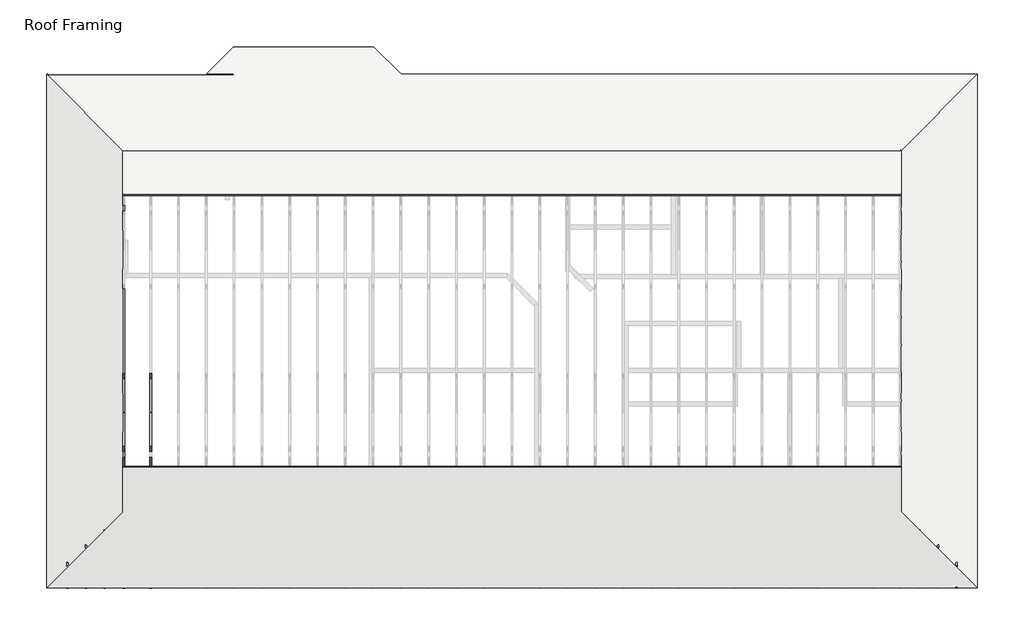
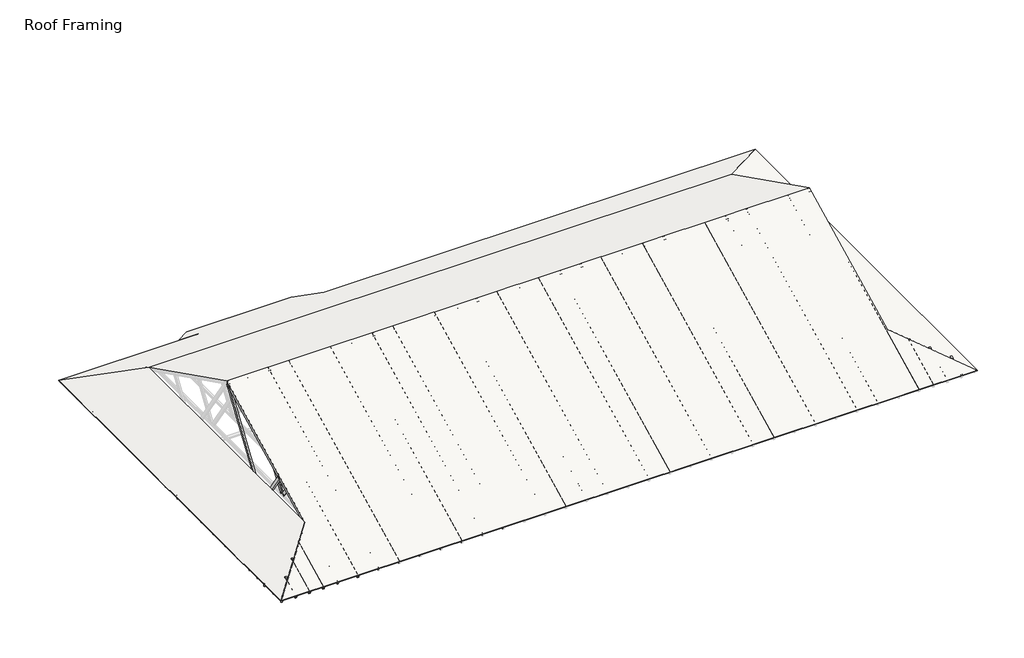
# One storey, part 1 of 7: 42 beams, 4 members, 4 roofs.
"""IFC4 building model written with IfcOpenShell, lengths in millimetres."""

import ifcopenshell
import ifcopenshell.guid

model = None  # the IFC model being written
_history = None  # IfcOwnerHistory: only IFC2X3 demands one
_inside = {}  # id of a spatial element -> (the spatial element, [elements in it])
_under = {}  # id of a project, library or spatial element -> (it, [spatial elements below it])
_declared = {}  # id of a project -> (the project, [libraries it declares])
_typed = {}  # id of a type object -> (the type object, [elements of that type])
_made_of = {}  # id of a material, layer set ... -> (it, [elements and type objects made of it])


def new_model(schema):
    """Start an empty IFC model of exactly this schema.

    Asked for "IFC4X3", IfcOpenShell would pick the latest addendum, in which some entities
    have other attributes; the version numbers below select the first issue.
    IFC2X3 requires an IfcOwnerHistory on every rooted entity: one is made here for all.
    """
    global model, _history
    if schema == "IFC4X3":
        model = ifcopenshell.file(schema_version=(4, 3, 0, 0))
    else:
        model = ifcopenshell.file(schema=schema)
    _inside.clear()
    _under.clear()
    _declared.clear()
    _typed.clear()
    _made_of.clear()
    _history = None
    if model.schema == "IFC2X3":
        org = make("IfcOrganization", Name="unknown")
        user = make(
            "IfcPersonAndOrganization",
            ThePerson=make("IfcPerson", FamilyName="unknown"),
            TheOrganization=org,
        )
        app = make(
            "IfcApplication",
            ApplicationDeveloper=org,
            Version="unknown",
            ApplicationFullName="unknown",
            ApplicationIdentifier="unknown",
        )
        _history = make(
            "IfcOwnerHistory",
            OwningUser=user,
            OwningApplication=app,
            ChangeAction="ADDED",
            CreationDate=0,
        )
    return model


def make(cls, **values):
    """One entity of the class cls with the attributes given. An attribute that is None is left unset."""
    return model.create_entity(
        cls, **{name: value for name, value in values.items() if value is not None}
    )


def rooted(cls, **values):
    """An entity with a GlobalId (a new one), such as an element, a storey or a relation."""
    return make(cls, GlobalId=ifcopenshell.guid.new(), OwnerHistory=_history, **values)


def si_unit(unit_type, name, prefix=None):
    """IfcSIUnit, for example si_unit("LENGTHUNIT", "METRE", prefix="MILLI")."""
    return make("IfcSIUnit", UnitType=unit_type, Prefix=prefix, Name=name)


def assignment(units):
    """IfcUnitAssignment: the units of a project."""
    return None if units is None else make("IfcUnitAssignment", Units=units)


def point(xyz):
    """IfcCartesianPoint."""
    return None if xyz is None else make("IfcCartesianPoint", Coordinates=xyz)


def direction(xyz):
    """IfcDirection."""
    return None if xyz is None else make("IfcDirection", DirectionRatios=xyz)


def frame(location, z_axis=None, x_axis=None):
    """IfcAxis2Placement3D, a coordinate frame: its origin and axes. An axis left out is left unset."""
    return make(
        "IfcAxis2Placement3D",
        Location=point(location),
        Axis=direction(z_axis),
        RefDirection=direction(x_axis),
    )


def origin():
    """The frame at (0, 0, 0) with its axes left unset."""
    return frame((0.0, 0.0, 0.0))


def place(relative_to, where):
    """IfcLocalPlacement: puts the frame where relative to a parent placement (None: the world)."""
    return make(
        "IfcLocalPlacement", PlacementRelTo=relative_to, RelativePlacement=where
    )


def context(
    kind, dimensions, precision=None, world=None, true_north=None, identifier=None
):
    """IfcGeometricRepresentationContext, for example the 3D "Model" context."""
    return make(
        "IfcGeometricRepresentationContext",
        ContextIdentifier=identifier,
        ContextType=kind,
        CoordinateSpaceDimension=dimensions,
        Precision=precision,
        WorldCoordinateSystem=world,
        TrueNorth=true_north,
    )


def project(units=None, contexts=None):
    """IfcProject with its units and contexts."""
    return rooted(
        "IfcProject",
        Name="project",
        RepresentationContexts=contexts,
        UnitsInContext=assignment(units),
    )


def spatial(cls, under=None, at=None, **own):
    """A site, building, storey or space (cls), placed at a placement, below another one or the project."""
    s = rooted(cls, ObjectPlacement=at, **own)
    if under is not None:
        _under.setdefault(under.id(), (under, []))[1].append(s)
    return s


def polyline(points):
    """IfcPolyline through the points."""
    return make("IfcPolyline", Points=[point(p) for p in points])


def outline(outer, holes=None, kind="AREA"):
    """IfcArbitraryClosedProfileDef: a profile drawn as a closed curve; with holes, ...WithVoids."""
    if holes is None:
        return make("IfcArbitraryClosedProfileDef", ProfileType=kind, OuterCurve=outer)
    return make(
        "IfcArbitraryProfileDefWithVoids",
        ProfileType=kind,
        OuterCurve=outer,
        InnerCurves=holes,
    )


def extrude(swept, where, along, depth):
    """IfcExtrudedAreaSolid: the profile swept, set in the frame where, extruded along a direction by depth."""
    return make(
        "IfcExtrudedAreaSolid",
        SweptArea=swept,
        Position=where,
        ExtrudedDirection=direction(along),
        Depth=depth,
    )


def faces_of(points, faces, orient=None, outer=None):
    """IfcFace entities. A face is a list of loops; a loop is a list of indices into points, from 0.

    orient and outer hold one flag for each loop. By default every Orientation is true, the
    first loop of a face is its IfcFaceOuterBound and the others are IfcFaceBound.
    """
    made = []
    for i, loops in enumerate(faces):
        bounds = []
        for j, loop in enumerate(loops):
            is_outer = j == 0 if outer is None else outer[i][j]
            bounds.append(
                make(
                    "IfcFaceOuterBound" if is_outer else "IfcFaceBound",
                    Bound=make("IfcPolyLoop", Polygon=[points[k] for k in loop]),
                    Orientation=True if orient is None else orient[i][j],
                )
            )
        made.append(make("IfcFace", Bounds=bounds))
    return made


def faceted_brep(points, faces, orient=None, outer=None, voids=None):
    """IfcFacetedBrep: a solid bounded by flat faces; with voids (closed shells), ...WithVoids."""
    shared = [point(p) for p in points]
    hull = make("IfcClosedShell", CfsFaces=faces_of(shared, faces, orient, outer))
    if voids is None:
        return make("IfcFacetedBrep", Outer=hull)
    return make(
        "IfcFacetedBrepWithVoids",
        Outer=hull,
        Voids=[
            make(cls, CfsFaces=faces_of(shared, fs, o, b)) for cls, fs, o, b in voids
        ],
    )


def shape(context_of_items, identifier, shape_type, items):
    """IfcShapeRepresentation: the items that make up one representation, for example the "Body"."""
    return make(
        "IfcShapeRepresentation",
        ContextOfItems=context_of_items,
        RepresentationIdentifier=identifier,
        RepresentationType=shape_type,
        Items=items,
    )


def source(mapping_origin, context_of_items, identifier, shape_type, items):
    """IfcRepresentationMap: a shape defined once, which mapped items show again and again."""
    return make(
        "IfcRepresentationMap",
        MappingOrigin=mapping_origin,
        MappedRepresentation=shape(context_of_items, identifier, shape_type, items),
    )


def transform(
    local_origin,
    x_axis=None,
    y_axis=None,
    z_axis=None,
    scale=None,
    scale2=None,
    scale3=None,
    uniform=True,
):
    """IfcCartesianTransformationOperator3D, or its non-uniform kind. x_axis, y_axis, z_axis: its Axis1, 2, 3."""
    if uniform:
        return make(
            "IfcCartesianTransformationOperator3D",
            Axis1=direction(x_axis),
            Axis2=direction(y_axis),
            LocalOrigin=point(local_origin),
            Scale=scale,
            Axis3=direction(z_axis),
        )
    return make(
        "IfcCartesianTransformationOperator3DnonUniform",
        Axis1=direction(x_axis),
        Axis2=direction(y_axis),
        LocalOrigin=point(local_origin),
        Scale=scale,
        Axis3=direction(z_axis),
        Scale2=scale2,
        Scale3=scale3,
    )


def mapped(mapping_source, mapping_target):
    """IfcMappedItem: shows the shape of a source again, moved by a transform."""
    return make(
        "IfcMappedItem", MappingSource=mapping_source, MappingTarget=mapping_target
    )


def made_of(thing, what):
    """Note that an element or type object is made of a material, layer set ...; save() writes the relation."""
    if what is not None:
        _made_of.setdefault(what.id(), (what, []))[1].append(thing)
    return thing


def element(
    cls,
    number,
    at=None,
    inside=None,
    cuts=None,
    type_object=None,
    material=None,
    context=None,
    identifier="Body",
    shape_type=None,
    held_by="IfcProductDefinitionShape",
    body=None,
    shapes=None,
    **own,
):
    """One element of the class cls, such as IfcWall. Its Tag is "e" and its number.

    at: its placement. inside: the storey or other place that contains it. cuts: it is an
    opening in that element (IfcRelVoidsElement). A single representation is given by context,
    identifier, shape_type and body (its items); several are given by shapes. held_by: the class
    of the entity that holds the representations. save() writes the other relations.
    """
    e = rooted(cls, Tag="e%d" % number, ObjectPlacement=at, **own)
    if body is not None:
        shapes = [shape(context, identifier, shape_type, body)]
    if shapes is not None:
        e.Representation = make(held_by, Representations=shapes)
    if inside is not None:
        _inside.setdefault(inside.id(), (inside, []))[1].append(e)
    if cuts is not None:
        rooted(
            "IfcRelVoidsElement", RelatingBuildingElement=cuts, RelatedOpeningElement=e
        )
    if type_object is not None:
        _typed.setdefault(type_object.id(), (type_object, []))[1].append(e)
    return made_of(e, material)


def aggregate(whole, parts):
    """IfcRelAggregates: a whole, such as a stair, and the parts it consists of."""
    return rooted("IfcRelAggregates", RelatingObject=whole, RelatedObjects=parts)


def save(model, path):
    """Write the relations noted so far, then the file.

    IfcRelAggregates (storeys below a building ...), IfcRelContainedInSpatialStructure (elements
    in a storey), IfcRelDefinesByType, IfcRelAssociatesMaterial and IfcRelDeclares: one each for
    every whole, place, type object, material and project.
    """
    for whole, parts in _under.values():
        aggregate(whole, parts)
    for where, things in _inside.values():
        rooted(
            "IfcRelContainedInSpatialStructure",
            RelatedElements=things,
            RelatingStructure=where,
        )
    for kind, things in _typed.values():
        rooted("IfcRelDefinesByType", RelatedObjects=things, RelatingType=kind)
    for what, things in _made_of.values():
        rooted("IfcRelAssociatesMaterial", RelatedObjects=things, RelatingMaterial=what)
    for by, libraries in _declared.values():
        rooted("IfcRelDeclares", RelatingContext=by, RelatedDefinitions=libraries)
    model.write(path)


def dimension_lumber_3c164bda(model_context):
    return source(origin(), model_context, "Body", "SweptSolid", [
        extrude(outline(polyline([(4638.675, -19.05), (-5762.625, -19.05), (-5762.625, 19.05), (4638.675, 19.05), (4638.675, -19.05)])), frame((0.0, 0.0, -44.45), z_axis=(0.0, 0.0, 1.0), x_axis=(1.0, 0.0, 0.0)), (0.0, 0.0, 1.0), 88.9),
    ])


def dimension_lumber_70fa0837(model_context):
    return source(origin(), model_context, "Body", "SweptSolid", [
        extrude(outline(polyline([(1250.4988621, 19.05), (1250.4988621, -19.05), (-1214.6940206, -19.05), (-1214.6940206, 19.05), (1250.4988621, 19.05)])), frame((0.0, 0.0, -44.45), z_axis=(0.0, 0.0, 1.0), x_axis=(1.0, 0.0, 0.0)), (0.0, 0.0, 1.0), 88.9),
    ])


def dimension_lumber_c8f8d63a(model_context):
    return source(origin(), model_context, "Body", "SweptSolid", [
        extrude(outline(polyline([(5118.89375, 44.45), (5118.89375, -44.45), (-5118.89375, -44.45), (-5118.89375, 44.45), (5118.89375, 44.45)])), frame((0.0, 0.0, -19.05), z_axis=(0.0, 0.0, 1.0), x_axis=(1.0, 0.0, 0.0)), (0.0, 0.0, 1.0), 38.1),
    ])


def dimension_lumber_4f6bd669(model_context):
    return source(origin(), model_context, "Body", "SweptSolid", [
        extrude(outline(polyline([(5017.29375, 44.45), (5017.29375, -44.45), (-5144.29375, -44.45), (-5144.29375, 44.45), (5017.29375, 44.45)])), frame((0.0, 0.0, -19.05), z_axis=(0.0, 0.0, 1.0), x_axis=(1.0, 0.0, 0.0)), (0.0, 0.0, 1.0), 38.1),
    ])


model = new_model("IFC4")

# Units and contexts
model_context = context("Model", 3, world=origin())
ifc_project = project(units=[si_unit("LENGTHUNIT", "METRE", prefix="MILLI")], contexts=[model_context])

# Site, building, storey
site = spatial("IfcSite", under=ifc_project)
building = spatial("IfcBuilding", under=site)
storey = spatial("IfcBuildingStorey", under=building, Name="Roof Framing", Elevation=2768.6)

# Beams
placement = place(None, origin())
element("IfcBeam", 1, ObjectType="Dimension Lumber : Roof Lumbers", at=placement, inside=storey, context=model_context, shape_type="SweptSolid", body=[
    extrude(outline(polyline([(-5032.8152251, -4625.6040947), (-5032.8152251, -4663.7040947), (-6240.9027251, -4663.7040947), (-6240.9027251, -4625.6040947), (-5032.8152251, -4625.6040947)])), frame((0.0, 0.0, 2768.6), z_axis=(0.0, 0.0, 1.0), x_axis=(1.0, 0.0, 0.0)), (0.0, 0.0, 1.0), 88.9),
    extrude(outline(polyline([(2768.6, -5032.8152251), (2857.5, -5032.8152251), (2857.5, -6064.1385305), (2769.1179027, -6240.9027251), (2768.6, -6240.9027251), (2768.6, -5032.8152251)])), frame((0.0, -4663.7040947, 0.0), z_axis=(0.0, 1.0, 0.0), x_axis=(0.0, 0.0, 1.0)), (0.0, 0.0, 1.0), 38.1),
])
element("IfcBeam", 2, ObjectType="Dimension Lumber : Roof Lumbers", at=placement, inside=storey, context=model_context, shape_type="SweptSolid", body=[
    extrude(outline(polyline([(-5032.8152251, -4016.0040947), (-5032.8152251, -4054.1040947), (-6240.9027251, -4054.1040947), (-6240.9027251, -4016.0040947), (-5032.8152251, -4016.0040947)])), frame((0.0, 0.0, 2768.6), z_axis=(0.0, 0.0, 1.0), x_axis=(1.0, 0.0, 0.0)), (0.0, 0.0, 1.0), 88.9),
    extrude(outline(polyline([(2768.6, -5032.8152251), (2857.5, -5032.8152251), (2857.5, -6064.1385305), (2769.1179027, -6240.9027251), (2768.6, -6240.9027251), (2768.6, -5032.8152251)])), frame((0.0, -4054.1040947, 0.0), z_axis=(0.0, 1.0, 0.0), x_axis=(0.0, 0.0, 1.0)), (0.0, 0.0, 1.0), 38.1),
])
element("IfcBeam", 3, ObjectType="Dimension Lumber : Roof Lumbers", at=placement, inside=storey, context=model_context, shape_type="SweptSolid", body=[
    extrude(outline(polyline([(-5032.8152251, -3406.4040947), (-5032.8152251, -3444.5040947), (-6240.9027251, -3444.5040947), (-6240.9027251, -3406.4040947), (-5032.8152251, -3406.4040947)])), frame((0.0, 0.0, 2768.6), z_axis=(0.0, 0.0, 1.0), x_axis=(1.0, 0.0, 0.0)), (0.0, 0.0, 1.0), 88.9),
    extrude(outline(polyline([(2768.6, -5032.8152251), (2857.5, -5032.8152251), (2857.5, -6064.1385305), (2769.1179027, -6240.9027251), (2768.6, -6240.9027251), (2768.6, -5032.8152251)])), frame((0.0, -3444.5040947, 0.0), z_axis=(0.0, 1.0, 0.0), x_axis=(0.0, 0.0, 1.0)), (0.0, 0.0, 1.0), 38.1),
])
element("IfcBeam", 4, ObjectType="Dimension Lumber : Roof Lumbers", at=placement, inside=storey, context=model_context, shape_type="SweptSolid", body=[
    extrude(outline(polyline([(-5032.8152251, -2796.8040947), (-5032.8152251, -2834.9040947), (-6240.9027251, -2834.9040947), (-6240.9027251, -2796.8040947), (-5032.8152251, -2796.8040947)])), frame((0.0, 0.0, 2768.6), z_axis=(0.0, 0.0, 1.0), x_axis=(1.0, 0.0, 0.0)), (0.0, 0.0, 1.0), 88.9),
    extrude(outline(polyline([(2768.6, -5032.8152251), (2857.5, -5032.8152251), (2857.5, -6064.1385305), (2769.1179027, -6240.9027251), (2768.6, -6240.9027251), (2768.6, -5032.8152251)])), frame((0.0, -2834.9040947, 0.0), z_axis=(0.0, 1.0, 0.0), x_axis=(0.0, 0.0, 1.0)), (0.0, 0.0, 1.0), 38.1),
])
element("IfcBeam", 5, ObjectType="Dimension Lumber : Roof Lumbers", at=placement, inside=storey, context=model_context, shape_type="SweptSolid", body=[
    extrude(outline(polyline([(-5032.8152251, -2187.2040947), (-5032.8152251, -2225.3040947), (-6240.9027251, -2225.3040947), (-6240.9027251, -2187.2040947), (-5032.8152251, -2187.2040947)])), frame((0.0, 0.0, 2768.6), z_axis=(0.0, 0.0, 1.0), x_axis=(1.0, 0.0, 0.0)), (0.0, 0.0, 1.0), 88.9),
    extrude(outline(polyline([(2768.6, -5032.8152251), (2857.5, -5032.8152251), (2857.5, -6064.1385305), (2769.1179027, -6240.9027251), (2768.6, -6240.9027251), (2768.6, -5032.8152251)])), frame((0.0, -2225.3040947, 0.0), z_axis=(0.0, 1.0, 0.0), x_axis=(0.0, 0.0, 1.0)), (0.0, 0.0, 1.0), 38.1),
])
element("IfcBeam", 6, ObjectType="Dimension Lumber : Roof Lumbers", at=placement, inside=storey, context=model_context, shape_type="SweptSolid", body=[
    extrude(outline(polyline([(-5032.8152251, -1577.6040947), (-5032.8152251, -1615.7040947), (-6240.9027251, -1615.7040947), (-6240.9027251, -1577.6040947), (-5032.8152251, -1577.6040947)])), frame((0.0, 0.0, 2768.6), z_axis=(0.0, 0.0, 1.0), x_axis=(1.0, 0.0, 0.0)), (0.0, 0.0, 1.0), 88.9),
    extrude(outline(polyline([(2768.6, -5032.8152251), (2857.5, -5032.8152251), (2857.5, -6064.1385305), (2769.1179027, -6240.9027251), (2768.6, -6240.9027251), (2768.6, -5032.8152251)])), frame((0.0, -1615.7040947, 0.0), z_axis=(0.0, 1.0, 0.0), x_axis=(0.0, 0.0, 1.0)), (0.0, 0.0, 1.0), 38.1),
])
element("IfcBeam", 7, ObjectType="Dimension Lumber : Roof Lumbers", at=placement, inside=storey, context=model_context, shape_type="SweptSolid", body=[
    extrude(outline(polyline([(-5032.8152251, -968.0040947), (-5032.8152251, -1006.1040947), (-6240.9027251, -1006.1040947), (-6240.9027251, -968.0040947), (-5032.8152251, -968.0040947)])), frame((0.0, 0.0, 2768.6), z_axis=(0.0, 0.0, 1.0), x_axis=(1.0, 0.0, 0.0)), (0.0, 0.0, 1.0), 88.9),
    extrude(outline(polyline([(2768.6, -5032.8152251), (2857.5, -5032.8152251), (2857.5, -6064.1385305), (2769.1179027, -6240.9027251), (2768.6, -6240.9027251), (2768.6, -5032.8152251)])), frame((0.0, -1006.1040947, 0.0), z_axis=(0.0, 1.0, 0.0), x_axis=(0.0, 0.0, 1.0)), (0.0, 0.0, 1.0), 38.1),
])
element("IfcBeam", 8, ObjectType="Dimension Lumber : Roof Lumbers", at=placement, inside=storey, context=model_context, shape_type="SweptSolid", body=[
    extrude(outline(polyline([(-5032.8152251, -358.4040947), (-5032.8152251, -396.5040947), (-6240.9027251, -396.5040947), (-6240.9027251, -358.4040947), (-5032.8152251, -358.4040947)])), frame((0.0, 0.0, 2768.6), z_axis=(0.0, 0.0, 1.0), x_axis=(1.0, 0.0, 0.0)), (0.0, 0.0, 1.0), 88.9),
    extrude(outline(polyline([(2768.6, -5032.8152251), (2857.5, -5032.8152251), (2857.5, -6064.1385305), (2769.1179027, -6240.9027251), (2768.6, -6240.9027251), (2768.6, -5032.8152251)])), frame((0.0, -396.5040947, 0.0), z_axis=(0.0, 1.0, 0.0), x_axis=(0.0, 0.0, 1.0)), (0.0, 0.0, 1.0), 38.1),
])
element("IfcBeam", 9, ObjectType="Dimension Lumber : Roof Lumbers", at=placement, inside=storey, context=model_context, shape_type="Brep", body=[
    faceted_brep([(-5458.2652251, -5041.9472419, 3273.9083007), (-5420.1652251, -5041.9472419, 3273.9083007), (-5420.1652251, -5002.1899532, 3194.3937234), (-5458.2652251, -5002.1899532, 3194.3937234), (-5458.2652251, -6329.0380921, 2630.3628756), (-5458.2652251, -6289.2808035, 2550.8482983), (-5420.1652251, -6289.2808035, 2550.8482983), (-5420.1652251, -6329.0380921, 2630.3628756)], [[[0, 1, 2, 3]], [[4, 5, 6, 7]], [[1, 0, 4, 7]], [[2, 1, 7, 6]], [[3, 2, 6, 5]], [[0, 3, 5, 4]]]),
    faceted_brep([(-5458.2652251, -6329.0380921, 2630.3628756), (-5458.2652251, -6289.2808035, 2550.8482983), (-5420.1652251, -6289.2808035, 2550.8482983), (-5420.1652251, -6329.0380921, 2630.3628756), (-5458.2652251, -5097.0448631, 3146.9662685), (-5458.2652251, -5097.0448631, 3246.3594901), (-5420.1652251, -5058.9448631, 3166.0162685), (-5420.1652251, -5058.9448631, 3265.4094901)], [[[0, 1, 2, 3]], [[4, 1, 0, 5]], [[6, 2, 1, 4]], [[7, 3, 2, 6]], [[5, 0, 3, 7]], [[5, 7, 6, 4]]]),
    faceted_brep([(-5458.2652251, -6329.0380921, 2630.3628756), (-5458.2652251, -6296.1597793, 2564.60625), (-5420.1652251, -6296.1597793, 2564.60625), (-5420.1652251, -6329.0380921, 2630.3628756), (-5458.2652251, -5097.0448631, 3146.9662685), (-5458.2652251, -6261.7649001, 2564.60625), (-5458.2652251, -5097.0448631, 3246.3594901), (-5420.1652251, -5058.9448631, 3265.4094901), (-5420.1652251, -6261.7649001, 2564.60625), (-5420.1652251, -5058.9448631, 3166.0162685)], [[[0, 1, 2, 3]], [[4, 5, 1, 0, 6]], [[7, 3, 2, 8, 9]], [[6, 0, 3, 7]], [[9, 8, 5, 4]], [[6, 7, 9, 4]], [[2, 1, 5, 8]]]),
    faceted_brep([(-5458.2652251, -5097.0448631, 3146.9662685), (-5458.2652251, -6261.7649001, 2564.60625), (-5458.2652251, -6282.9540947, 2564.60625), (-5458.2652251, -6282.9540947, 2653.4048743), (-5458.2652251, -5097.0448631, 3246.3594901), (-5420.1652251, -5058.9448631, 3166.0162685), (-5420.1652251, -6261.7649001, 2564.60625), (-5420.1652251, -6282.9540947, 2564.60625), (-5420.1652251, -6282.9540947, 2653.4048743), (-5420.1652251, -5058.9448631, 3265.4094901)], [[[0, 1, 2, 3, 4]], [[5, 6, 1, 0]], [[2, 1, 6, 7]], [[4, 3, 8, 9]], [[4, 9, 5, 0]], [[9, 8, 7, 6, 5]], [[3, 2, 7, 8]]]),
])
element("IfcBeam", 10, ObjectType="Dimension Lumber : Roof Lumbers", at=placement, inside=storey, context=model_context, shape_type="Brep", body=[
    faceted_brep([(-5864.6652251, -5385.152618, 3102.3056127), (-5826.5652251, -5385.152618, 3102.3056127), (-5826.5652251, -5345.3953294, 3022.7910354), (-5864.6652251, -5345.3953294, 3022.7910354), (-5864.6652251, -6329.0380921, 2630.3628756), (-5864.6652251, -6289.2808035, 2550.8482983), (-5826.5652251, -6289.2808035, 2550.8482983), (-5826.5652251, -6329.0380921, 2630.3628756)], [[[0, 1, 2, 3]], [[4, 5, 6, 7]], [[1, 0, 4, 7]], [[2, 1, 7, 6]], [[3, 2, 6, 5]], [[0, 3, 5, 4]]]),
    faceted_brep([(-5864.6652251, -6329.0380921, 2630.3628756), (-5864.6652251, -6289.2808035, 2550.8482983), (-5826.5652251, -6289.2808035, 2550.8482983), (-5826.5652251, -6329.0380921, 2630.3628756), (-5864.6652251, -5503.4448631, 2943.7662685), (-5864.6652251, -5503.4448631, 3043.1594901), (-5826.5652251, -5465.3448631, 2962.8162685), (-5826.5652251, -5465.3448631, 3062.2094901)], [[[0, 1, 2, 3]], [[4, 1, 0, 5]], [[6, 2, 1, 4]], [[7, 3, 2, 6]], [[5, 0, 3, 7]], [[5, 7, 6, 4]]]),
    faceted_brep([(-5864.6652251, -6329.0380921, 2630.3628756), (-5864.6652251, -6296.1597793, 2564.60625), (-5826.5652251, -6296.1597793, 2564.60625), (-5826.5652251, -6329.0380921, 2630.3628756), (-5864.6652251, -5503.4448631, 2943.7662685), (-5864.6652251, -6261.7649001, 2564.60625), (-5864.6652251, -5503.4448631, 3043.1594901), (-5826.5652251, -5465.3448631, 3062.2094901), (-5826.5652251, -6261.7649001, 2564.60625), (-5826.5652251, -5465.3448631, 2962.8162685)], [[[0, 1, 2, 3]], [[4, 5, 1, 0, 6]], [[7, 3, 2, 8, 9]], [[6, 0, 3, 7]], [[9, 8, 5, 4]], [[6, 7, 9, 4]], [[2, 1, 5, 8]]]),
    faceted_brep([(-5864.6652251, -5503.4448631, 2943.7662685), (-5864.6652251, -6261.7649001, 2564.60625), (-5864.6652251, -6282.9540947, 2564.60625), (-5864.6652251, -6282.9540947, 2653.4048743), (-5864.6652251, -5503.4448631, 3043.1594901), (-5826.5652251, -5465.3448631, 2962.8162685), (-5826.5652251, -6261.7649001, 2564.60625), (-5826.5652251, -6282.9540947, 2564.60625), (-5826.5652251, -6282.9540947, 2653.4048743), (-5826.5652251, -5465.3448631, 3062.2094901)], [[[0, 1, 2, 3, 4]], [[5, 6, 1, 0]], [[2, 1, 6, 7]], [[4, 3, 8, 9]], [[4, 9, 5, 0]], [[9, 8, 7, 6, 5]], [[3, 2, 7, 8]]]),
])
element("IfcBeam", 11, ObjectType="Dimension Lumber : Roof Lumbers", at=placement, inside=storey, context=model_context, shape_type="Brep", body=[
    faceted_brep([(-6271.0652251, -5771.3662791, 2909.1987821), (-6232.9652251, -5771.3662791, 2909.1987821), (-6232.9652251, -5731.6089904, 2829.6842048), (-6271.0652251, -5731.6089904, 2829.6842048), (-6271.0652251, -6329.0380921, 2630.3628756), (-6271.0652251, -6289.2808035, 2550.8482983), (-6232.9652251, -6289.2808035, 2550.8482983), (-6232.9652251, -6329.0380921, 2630.3628756)], [[[0, 1, 2, 3]], [[4, 5, 6, 7]], [[1, 0, 4, 7]], [[2, 1, 7, 6]], [[3, 2, 6, 5]], [[0, 3, 5, 4]]]),
    faceted_brep([(-6271.0652251, -6329.0380921, 2630.3628756), (-6271.0652251, -6289.2808035, 2550.8482983), (-6232.9652251, -6289.2808035, 2550.8482983), (-6232.9652251, -6329.0380921, 2630.3628756), (-6271.0652251, -5909.8448631, 2740.5662685), (-6271.0652251, -5909.8448631, 2839.9594901), (-6232.9652251, -5871.7448631, 2759.6162685), (-6232.9652251, -5871.7448631, 2859.0094901)], [[[0, 1, 2, 3]], [[4, 1, 0, 5]], [[6, 2, 1, 4]], [[7, 3, 2, 6]], [[5, 0, 3, 7]], [[5, 7, 6, 4]]]),
    faceted_brep([(-6271.0652251, -6329.0380921, 2630.3628756), (-6271.0652251, -6296.1597793, 2564.60625), (-6232.9652251, -6296.1597793, 2564.60625), (-6232.9652251, -6329.0380921, 2630.3628756), (-6271.0652251, -5909.8448631, 2740.5662685), (-6271.0652251, -6261.7649001, 2564.60625), (-6271.0652251, -5909.8448631, 2839.9594901), (-6232.9652251, -5871.7448631, 2859.0094901), (-6232.9652251, -6261.7649001, 2564.60625), (-6232.9652251, -5871.7448631, 2759.6162685)], [[[0, 1, 2, 3]], [[4, 5, 1, 0, 6]], [[7, 3, 2, 8, 9]], [[6, 0, 3, 7]], [[9, 8, 5, 4]], [[6, 7, 9, 4]], [[2, 1, 5, 8]]]),
    faceted_brep([(-6271.0652251, -5909.8448631, 2740.5662685), (-6271.0652251, -6261.7649001, 2564.60625), (-6271.0652251, -6282.9540947, 2564.60625), (-6271.0652251, -6282.9540947, 2653.4048743), (-6271.0652251, -5909.8448631, 2839.9594901), (-6232.9652251, -5871.7448631, 2759.6162685), (-6232.9652251, -6261.7649001, 2564.60625), (-6232.9652251, -6282.9540947, 2564.60625), (-6232.9652251, -6282.9540947, 2653.4048743), (-6232.9652251, -5871.7448631, 2859.0094901)], [[[0, 1, 2, 3, 4]], [[5, 6, 1, 0]], [[2, 1, 6, 7]], [[4, 3, 8, 9]], [[4, 9, 5, 0]], [[9, 8, 7, 6, 5]], [[3, 2, 7, 8]]]),
])
dimension_lumber_shape = dimension_lumber_3c164bda(model_context)
element("IfcBeam", 12, ObjectType="Dimension Lumber : Roof Lumbers", at=placement, inside=storey, context=model_context, shape_type="MappedRepresentation", body=[
    mapped(dimension_lumber_shape, transform((-6271.0652251, -139.3290947, 2609.05625), x_axis=(0.0, 1.0, 0.0), y_axis=(-1.0, 0.0, 0.0), z_axis=(0.0, 0.0, 1.0))),
])
dimension_lumber_2_shape = dimension_lumber_70fa0837(model_context)
element("IfcBeam", 13, ObjectType="Dimension Lumber : Roof Lumbers", at=placement, inside=storey, context=model_context, shape_type="MappedRepresentation", body=[
    mapped(dimension_lumber_2_shape, transform((-5859.0415503, -5470.8804199, 3005.560175), x_axis=(0.6666666666666689, 0.666666666666668, 0.33333333333332643), y_axis=(-0.707106781186547, 0.707106781186548, 0.0), z_axis=(-0.23570226039551115, -0.2357022603955108, 0.9428090415820658))),
])
dimension_lumber_3_shape = dimension_lumber_c8f8d63a(model_context)
element("IfcBeam", 14, ObjectType="Dimension Lumber : Top Supporting Lumbers", at=placement, inside=storey, context=model_context, shape_type="MappedRepresentation", body=[
    mapped(dimension_lumber_3_shape, transform((-6196.4527251, -630.6603447, 2711.45), x_axis=(0.0, 1.0, 0.0), y_axis=(-1.0, 0.0, 0.0), z_axis=(0.0, 0.0, 1.0))),
])
dimension_lumber_4_shape = dimension_lumber_4f6bd669(model_context)
element("IfcBeam", 15, ObjectType="Dimension Lumber : Top Supporting Lumbers", at=placement, inside=storey, context=model_context, shape_type="MappedRepresentation", body=[
    mapped(dimension_lumber_4_shape, transform((-1134.7089751, -5705.1040947, 2749.55), x_axis=(-1.0, 0.0, 0.0), y_axis=(0.0, -1.0, 0.0), z_axis=(0.0, 0.0, 1.0))),
])
element("IfcBeam", 16, ObjectType="Dimension Lumber : Top Supporting Lumbers", at=placement, inside=storey, context=model_context, shape_type="MappedRepresentation", body=[
    mapped(dimension_lumber_4_shape, transform((-1134.7089751, -5705.1040947, 2711.45), x_axis=(-1.0, 0.0, 0.0), y_axis=(0.0, -1.0, 0.0), z_axis=(0.0, 0.0, 1.0))),
])
element("IfcBeam", 17, ObjectType="Dimension Lumber : 2x4 Blocking", at=placement, inside=storey, context=model_context, shape_type="SweptSolid", body=[
    extrude(outline(polyline([(-6671.1152251, -4663.7040947), (-6671.1152251, -4625.6040947), (-6290.1152251, -4625.6040947), (-6290.1152251, -4663.7040947), (-6671.1152251, -4663.7040947)])), frame((0.0, 0.0, 2564.60625), z_axis=(0.0, 0.0, 1.0), x_axis=(1.0, 0.0, 0.0)), (0.0, 0.0, 1.0), 88.9),
    extrude(outline(polyline([(2564.60625, -6649.9260305), (2564.60625, -6290.1152251), (2653.50625, -6290.1152251), (2653.50625, -6472.1260305), (2564.60625, -6649.9260305)])), frame((0.0, -4663.7040947, 0.0), z_axis=(0.0, 1.0, 0.0), x_axis=(0.0, 0.0, 1.0)), (0.0, 0.0, 1.0), 38.1),
])
element("IfcBeam", 18, ObjectType="Dimension Lumber : 2x4 Blocking", at=placement, inside=storey, context=model_context, shape_type="SweptSolid", body=[
    extrude(outline(polyline([(-6671.1152251, -4054.1040947), (-6671.1152251, -4016.0040947), (-6290.1152251, -4016.0040947), (-6290.1152251, -4054.1040947), (-6671.1152251, -4054.1040947)])), frame((0.0, 0.0, 2564.60625), z_axis=(0.0, 0.0, 1.0), x_axis=(1.0, 0.0, 0.0)), (0.0, 0.0, 1.0), 88.9),
    extrude(outline(polyline([(2564.60625, -6649.9260305), (2564.60625, -6290.1152251), (2653.50625, -6290.1152251), (2653.50625, -6472.1260305), (2564.60625, -6649.9260305)])), frame((0.0, -4054.1040947, 0.0), z_axis=(0.0, 1.0, 0.0), x_axis=(0.0, 0.0, 1.0)), (0.0, 0.0, 1.0), 38.1),
])
element("IfcBeam", 19, ObjectType="Dimension Lumber : 2x4 Blocking", at=placement, inside=storey, context=model_context, shape_type="SweptSolid", body=[
    extrude(outline(polyline([(-6671.1152251, -3444.5040947), (-6671.1152251, -3406.4040947), (-6290.1152251, -3406.4040947), (-6290.1152251, -3444.5040947), (-6671.1152251, -3444.5040947)])), frame((0.0, 0.0, 2564.60625), z_axis=(0.0, 0.0, 1.0), x_axis=(1.0, 0.0, 0.0)), (0.0, 0.0, 1.0), 88.9),
    extrude(outline(polyline([(2564.60625, -6649.9260305), (2564.60625, -6290.1152251), (2653.50625, -6290.1152251), (2653.50625, -6472.1260305), (2564.60625, -6649.9260305)])), frame((0.0, -3444.5040947, 0.0), z_axis=(0.0, 1.0, 0.0), x_axis=(0.0, 0.0, 1.0)), (0.0, 0.0, 1.0), 38.1),
])
element("IfcBeam", 20, ObjectType="Dimension Lumber : 2x4 Blocking", at=placement, inside=storey, context=model_context, shape_type="SweptSolid", body=[
    extrude(outline(polyline([(-6671.1152251, -2834.9040947), (-6671.1152251, -2796.8040947), (-6290.1152251, -2796.8040947), (-6290.1152251, -2834.9040947), (-6671.1152251, -2834.9040947)])), frame((0.0, 0.0, 2564.60625), z_axis=(0.0, 0.0, 1.0), x_axis=(1.0, 0.0, 0.0)), (0.0, 0.0, 1.0), 88.9),
    extrude(outline(polyline([(2564.60625, -6649.9260305), (2564.60625, -6290.1152251), (2653.50625, -6290.1152251), (2653.50625, -6472.1260305), (2564.60625, -6649.9260305)])), frame((0.0, -2834.9040947, 0.0), z_axis=(0.0, 1.0, 0.0), x_axis=(0.0, 0.0, 1.0)), (0.0, 0.0, 1.0), 38.1),
])
element("IfcBeam", 21, ObjectType="Dimension Lumber : 2x4 Blocking", at=placement, inside=storey, context=model_context, shape_type="SweptSolid", body=[
    extrude(outline(polyline([(-6671.1152251, -2225.3040947), (-6671.1152251, -2187.2040947), (-6290.1152251, -2187.2040947), (-6290.1152251, -2225.3040947), (-6671.1152251, -2225.3040947)])), frame((0.0, 0.0, 2564.60625), z_axis=(0.0, 0.0, 1.0), x_axis=(1.0, 0.0, 0.0)), (0.0, 0.0, 1.0), 88.9),
    extrude(outline(polyline([(2564.60625, -6649.9260305), (2564.60625, -6290.1152251), (2653.50625, -6290.1152251), (2653.50625, -6472.1260305), (2564.60625, -6649.9260305)])), frame((0.0, -2225.3040947, 0.0), z_axis=(0.0, 1.0, 0.0), x_axis=(0.0, 0.0, 1.0)), (0.0, 0.0, 1.0), 38.1),
])
element("IfcBeam", 22, ObjectType="Dimension Lumber : 2x4 Blocking", at=placement, inside=storey, context=model_context, shape_type="SweptSolid", body=[
    extrude(outline(polyline([(-6671.1152251, -1615.7040947), (-6671.1152251, -1577.6040947), (-6290.1152251, -1577.6040947), (-6290.1152251, -1615.7040947), (-6671.1152251, -1615.7040947)])), frame((0.0, 0.0, 2564.60625), z_axis=(0.0, 0.0, 1.0), x_axis=(1.0, 0.0, 0.0)), (0.0, 0.0, 1.0), 88.9),
    extrude(outline(polyline([(2564.60625, -6649.9260305), (2564.60625, -6290.1152251), (2653.50625, -6290.1152251), (2653.50625, -6472.1260305), (2564.60625, -6649.9260305)])), frame((0.0, -1615.7040947, 0.0), z_axis=(0.0, 1.0, 0.0), x_axis=(0.0, 0.0, 1.0)), (0.0, 0.0, 1.0), 38.1),
])
element("IfcBeam", 23, ObjectType="Dimension Lumber : 2x4 Blocking", at=placement, inside=storey, context=model_context, shape_type="SweptSolid", body=[
    extrude(outline(polyline([(-6671.1152251, -1006.1040947), (-6671.1152251, -968.0040947), (-6290.1152251, -968.0040947), (-6290.1152251, -1006.1040947), (-6671.1152251, -1006.1040947)])), frame((0.0, 0.0, 2564.60625), z_axis=(0.0, 0.0, 1.0), x_axis=(1.0, 0.0, 0.0)), (0.0, 0.0, 1.0), 88.9),
    extrude(outline(polyline([(2564.60625, -6649.9260305), (2564.60625, -6290.1152251), (2653.50625, -6290.1152251), (2653.50625, -6472.1260305), (2564.60625, -6649.9260305)])), frame((0.0, -1006.1040947, 0.0), z_axis=(0.0, 1.0, 0.0), x_axis=(0.0, 0.0, 1.0)), (0.0, 0.0, 1.0), 38.1),
])
element("IfcBeam", 24, ObjectType="Dimension Lumber : 2x4 Blocking", at=placement, inside=storey, context=model_context, shape_type="SweptSolid", body=[
    extrude(outline(polyline([(-6671.1152251, -396.5040947), (-6671.1152251, -358.4040947), (-6290.1152251, -358.4040947), (-6290.1152251, -396.5040947), (-6671.1152251, -396.5040947)])), frame((0.0, 0.0, 2564.60625), z_axis=(0.0, 0.0, 1.0), x_axis=(1.0, 0.0, 0.0)), (0.0, 0.0, 1.0), 88.9),
    extrude(outline(polyline([(2564.60625, -6649.9260305), (2564.60625, -6290.1152251), (2653.50625, -6290.1152251), (2653.50625, -6472.1260305), (2564.60625, -6649.9260305)])), frame((0.0, -396.5040947, 0.0), z_axis=(0.0, 1.0, 0.0), x_axis=(0.0, 0.0, 1.0)), (0.0, 0.0, 1.0), 38.1),
])
element("IfcBeam", 25, ObjectType="Dimension Lumber : 2x4 Blocking", at=placement, inside=storey, context=model_context, shape_type="SweptSolid", body=[
    extrude(outline(polyline([(-175.0652251, -5901.9540947), (-136.9652251, -5901.9540947), (-136.9652251, -6282.9540947), (-175.0652251, -6282.9540947), (-175.0652251, -5901.9540947)])), frame((0.0, 0.0, 2564.60625), z_axis=(0.0, 0.0, 1.0), x_axis=(1.0, 0.0, 0.0)), (0.0, 0.0, 1.0), 88.9),
    extrude(outline(polyline([(-5901.9540947, 2653.50625), (-5901.9540947, 2564.60625), (-6261.7649001, 2564.60625), (-6083.9649001, 2653.50625), (-5901.9540947, 2653.50625)])), frame((-175.0652251, 0.0, 0.0), z_axis=(1.0, 0.0, 0.0), x_axis=(0.0, 1.0, 0.0)), (0.0, 0.0, 1.0), 38.1),
])
element("IfcBeam", 26, ObjectType="Dimension Lumber : 2x4 Blocking", at=placement, inside=storey, context=model_context, shape_type="SweptSolid", body=[
    extrude(outline(polyline([(-784.6652251, -5901.9540947), (-746.5652251, -5901.9540947), (-746.5652251, -6282.9540947), (-784.6652251, -6282.9540947), (-784.6652251, -5901.9540947)])), frame((0.0, 0.0, 2564.60625), z_axis=(0.0, 0.0, 1.0), x_axis=(1.0, 0.0, 0.0)), (0.0, 0.0, 1.0), 88.9),
    extrude(outline(polyline([(-5901.9540947, 2653.50625), (-5901.9540947, 2564.60625), (-6261.7649001, 2564.60625), (-6083.9649001, 2653.50625), (-5901.9540947, 2653.50625)])), frame((-784.6652251, 0.0, 0.0), z_axis=(1.0, 0.0, 0.0), x_axis=(0.0, 1.0, 0.0)), (0.0, 0.0, 1.0), 38.1),
])
element("IfcBeam", 27, ObjectType="Dimension Lumber : 2x4 Blocking", at=placement, inside=storey, context=model_context, shape_type="SweptSolid", body=[
    extrude(outline(polyline([(-1394.2652251, -5901.9540947), (-1356.1652251, -5901.9540947), (-1356.1652251, -6282.9540947), (-1394.2652251, -6282.9540947), (-1394.2652251, -5901.9540947)])), frame((0.0, 0.0, 2564.60625), z_axis=(0.0, 0.0, 1.0), x_axis=(1.0, 0.0, 0.0)), (0.0, 0.0, 1.0), 88.9),
    extrude(outline(polyline([(-5901.9540947, 2653.50625), (-5901.9540947, 2564.60625), (-6261.7649001, 2564.60625), (-6083.9649001, 2653.50625), (-5901.9540947, 2653.50625)])), frame((-1394.2652251, 0.0, 0.0), z_axis=(1.0, 0.0, 0.0), x_axis=(0.0, 1.0, 0.0)), (0.0, 0.0, 1.0), 38.1),
])
element("IfcBeam", 28, ObjectType="Dimension Lumber : 2x4 Blocking", at=placement, inside=storey, context=model_context, shape_type="SweptSolid", body=[
    extrude(outline(polyline([(-2003.8652251, -5901.9540947), (-1965.7652251, -5901.9540947), (-1965.7652251, -6282.9540947), (-2003.8652251, -6282.9540947), (-2003.8652251, -5901.9540947)])), frame((0.0, 0.0, 2564.60625), z_axis=(0.0, 0.0, 1.0), x_axis=(1.0, 0.0, 0.0)), (0.0, 0.0, 1.0), 88.9),
    extrude(outline(polyline([(-5901.9540947, 2653.50625), (-5901.9540947, 2564.60625), (-6261.7649001, 2564.60625), (-6083.9649001, 2653.50625), (-5901.9540947, 2653.50625)])), frame((-2003.8652251, 0.0, 0.0), z_axis=(1.0, 0.0, 0.0), x_axis=(0.0, 1.0, 0.0)), (0.0, 0.0, 1.0), 38.1),
])
element("IfcBeam", 29, ObjectType="Dimension Lumber : 2x4 Blocking", at=placement, inside=storey, context=model_context, shape_type="SweptSolid", body=[
    extrude(outline(polyline([(-2613.4652251, -5901.9540947), (-2575.3652251, -5901.9540947), (-2575.3652251, -6282.9540947), (-2613.4652251, -6282.9540947), (-2613.4652251, -5901.9540947)])), frame((0.0, 0.0, 2564.60625), z_axis=(0.0, 0.0, 1.0), x_axis=(1.0, 0.0, 0.0)), (0.0, 0.0, 1.0), 88.9),
    extrude(outline(polyline([(-5901.9540947, 2653.50625), (-5901.9540947, 2564.60625), (-6261.7649001, 2564.60625), (-6083.9649001, 2653.50625), (-5901.9540947, 2653.50625)])), frame((-2613.4652251, 0.0, 0.0), z_axis=(1.0, 0.0, 0.0), x_axis=(0.0, 1.0, 0.0)), (0.0, 0.0, 1.0), 38.1),
])
element("IfcBeam", 30, ObjectType="Dimension Lumber : 2x4 Blocking", at=placement, inside=storey, context=model_context, shape_type="SweptSolid", body=[
    extrude(outline(polyline([(-3223.0652251, -5901.9540947), (-3184.9652251, -5901.9540947), (-3184.9652251, -6282.9540947), (-3223.0652251, -6282.9540947), (-3223.0652251, -5901.9540947)])), frame((0.0, 0.0, 2564.60625), z_axis=(0.0, 0.0, 1.0), x_axis=(1.0, 0.0, 0.0)), (0.0, 0.0, 1.0), 88.9),
    extrude(outline(polyline([(-5901.9540947, 2653.50625), (-5901.9540947, 2564.60625), (-6261.7649001, 2564.60625), (-6083.9649001, 2653.50625), (-5901.9540947, 2653.50625)])), frame((-3223.0652251, 0.0, 0.0), z_axis=(1.0, 0.0, 0.0), x_axis=(0.0, 1.0, 0.0)), (0.0, 0.0, 1.0), 38.1),
])
element("IfcBeam", 31, ObjectType="Dimension Lumber : 2x4 Blocking", at=placement, inside=storey, context=model_context, shape_type="SweptSolid", body=[
    extrude(outline(polyline([(-3832.6652251, -5901.9540947), (-3794.5652251, -5901.9540947), (-3794.5652251, -6282.9540947), (-3832.6652251, -6282.9540947), (-3832.6652251, -5901.9540947)])), frame((0.0, 0.0, 2564.60625), z_axis=(0.0, 0.0, 1.0), x_axis=(1.0, 0.0, 0.0)), (0.0, 0.0, 1.0), 88.9),
    extrude(outline(polyline([(-5901.9540947, 2653.50625), (-5901.9540947, 2564.60625), (-6261.7649001, 2564.60625), (-6083.9649001, 2653.50625), (-5901.9540947, 2653.50625)])), frame((-3832.6652251, 0.0, 0.0), z_axis=(1.0, 0.0, 0.0), x_axis=(0.0, 1.0, 0.0)), (0.0, 0.0, 1.0), 38.1),
])
element("IfcBeam", 32, ObjectType="Dimension Lumber : 2x4 Blocking", at=placement, inside=storey, context=model_context, shape_type="SweptSolid", body=[
    extrude(outline(polyline([(-4442.2652251, -5901.9540947), (-4404.1652251, -5901.9540947), (-4404.1652251, -6282.9540947), (-4442.2652251, -6282.9540947), (-4442.2652251, -5901.9540947)])), frame((0.0, 0.0, 2564.60625), z_axis=(0.0, 0.0, 1.0), x_axis=(1.0, 0.0, 0.0)), (0.0, 0.0, 1.0), 88.9),
    extrude(outline(polyline([(-5901.9540947, 2653.50625), (-5901.9540947, 2564.60625), (-6261.7649001, 2564.60625), (-6083.9649001, 2653.50625), (-5901.9540947, 2653.50625)])), frame((-4442.2652251, 0.0, 0.0), z_axis=(1.0, 0.0, 0.0), x_axis=(0.0, 1.0, 0.0)), (0.0, 0.0, 1.0), 38.1),
])
element("IfcBeam", 33, ObjectType="Dimension Lumber : 2x4 Blocking", at=placement, inside=storey, context=model_context, shape_type="SweptSolid", body=[
    extrude(outline(polyline([(-5032.8152251, -5901.9540947), (-4994.7152251, -5901.9540947), (-4994.7152251, -6282.9540947), (-5032.8152251, -6282.9540947), (-5032.8152251, -5901.9540947)])), frame((0.0, 0.0, 2564.60625), z_axis=(0.0, 0.0, 1.0), x_axis=(1.0, 0.0, 0.0)), (0.0, 0.0, 1.0), 88.9),
    extrude(outline(polyline([(-5901.9540947, 2653.50625), (-5901.9540947, 2564.60625), (-6261.7649001, 2564.60625), (-6083.9649001, 2653.50625), (-5901.9540947, 2653.50625)])), frame((-5032.8152251, 0.0, 0.0), z_axis=(1.0, 0.0, 0.0), x_axis=(0.0, 1.0, 0.0)), (0.0, 0.0, 1.0), 38.1),
])
element("IfcBeam", 34, ObjectType="Dimension Lumber : 2x4 Blocking", at=placement, inside=storey, context=model_context, shape_type="SweptSolid", body=[
    extrude(outline(polyline([(-5458.2652251, -5901.9540947), (-5420.1652251, -5901.9540947), (-5420.1652251, -6289.2808035), (-5458.2652251, -6289.2808035), (-5458.2652251, -5901.9540947)])), frame((0.0, 0.0, 2564.60625), z_axis=(0.0, 0.0, 1.0), x_axis=(1.0, 0.0, 0.0)), (0.0, 0.0, 1.0), 88.9),
    extrude(outline(polyline([(-5901.9540947, 2653.50625), (-5901.9540947, 2564.60625), (-6261.7649001, 2564.60625), (-6083.9649001, 2653.50625), (-5901.9540947, 2653.50625)])), frame((-5458.2652251, 0.0, 0.0), z_axis=(1.0, 0.0, 0.0), x_axis=(0.0, 1.0, 0.0)), (0.0, 0.0, 1.0), 38.1),
])
element("IfcBeam", 35, ObjectType="Dimension Lumber : 2x4 Blocking", at=placement, inside=storey, context=model_context, shape_type="SweptSolid", body=[
    extrude(outline(polyline([(-5864.6652251, -5901.9540947), (-5826.5652251, -5901.9540947), (-5826.5652251, -6282.9540947), (-5864.6652251, -6282.9540947), (-5864.6652251, -5901.9540947)])), frame((0.0, 0.0, 2564.60625), z_axis=(0.0, 0.0, 1.0), x_axis=(1.0, 0.0, 0.0)), (0.0, 0.0, 1.0), 88.9),
    extrude(outline(polyline([(-5901.9540947, 2653.50625), (-5901.9540947, 2564.60625), (-6261.7649001, 2564.60625), (-6083.9649001, 2653.50625), (-5901.9540947, 2653.50625)])), frame((-5864.6652251, 0.0, 0.0), z_axis=(1.0, 0.0, 0.0), x_axis=(0.0, 1.0, 0.0)), (0.0, 0.0, 1.0), 38.1),
])
element("IfcBeam", 36, ObjectType="Dimension Lumber : 2x4 Blocking", at=placement, inside=storey, context=model_context, shape_type="SweptSolid", body=[
    extrude(outline(polyline([(-6271.0652251, -5901.9540947), (-6232.9652251, -5901.9540947), (-6232.9652251, -6282.9540947), (-6271.0652251, -6282.9540947), (-6271.0652251, -5901.9540947)])), frame((0.0, 0.0, 2564.60625), z_axis=(0.0, 0.0, 1.0), x_axis=(1.0, 0.0, 0.0)), (0.0, 0.0, 1.0), 88.9),
    extrude(outline(polyline([(-5901.9540947, 2653.50625), (-5901.9540947, 2564.60625), (-6261.7649001, 2564.60625), (-6083.9649001, 2653.50625), (-5901.9540947, 2653.50625)])), frame((-6271.0652251, 0.0, 0.0), z_axis=(1.0, 0.0, 0.0), x_axis=(0.0, 1.0, 0.0)), (0.0, 0.0, 1.0), 38.1),
])
element("IfcBeam", 37, ObjectType="Dimension Lumber : 2x4 Blocking", at=placement, inside=storey, context=model_context, shape_type="SweptSolid", body=[
    extrude(outline(polyline([(-6671.1152251, -5070.1040947), (-6671.1152251, -5032.0040947), (-6290.1152251, -5032.0040947), (-6290.1152251, -5070.1040947), (-6671.1152251, -5070.1040947)])), frame((0.0, 0.0, 2564.60625), z_axis=(0.0, 0.0, 1.0), x_axis=(1.0, 0.0, 0.0)), (0.0, 0.0, 1.0), 88.9),
    extrude(outline(polyline([(2564.60625, -6649.9260305), (2564.60625, -6290.1152251), (2653.50625, -6290.1152251), (2653.50625, -6472.1260305), (2564.60625, -6649.9260305)])), frame((0.0, -5070.1040947, 0.0), z_axis=(0.0, 1.0, 0.0), x_axis=(0.0, 0.0, 1.0)), (0.0, 0.0, 1.0), 38.1),
])
element("IfcBeam", 38, ObjectType="Dimension Lumber : 2x4 Blocking", at=placement, inside=storey, context=model_context, shape_type="SweptSolid", body=[
    extrude(outline(polyline([(-6690.1652251, -5476.5040947), (-6690.1652251, -5438.4040947), (-6290.1152251, -5438.4040947), (-6290.1152251, -5476.5040947), (-6690.1652251, -5476.5040947)])), frame((0.0, 0.0, 2564.60625), z_axis=(0.0, 0.0, 1.0), x_axis=(1.0, 0.0, 0.0)), (0.0, 0.0, 1.0), 88.9),
    extrude(outline(polyline([(2564.60625, -6649.9260305), (2564.60625, -6290.1152251), (2653.50625, -6290.1152251), (2653.50625, -6472.1260305), (2564.60625, -6649.9260305)])), frame((0.0, -5476.5040947, 0.0), z_axis=(0.0, 1.0, 0.0), x_axis=(0.0, 0.0, 1.0)), (0.0, 0.0, 1.0), 38.1),
])
element("IfcBeam", 39, ObjectType="Dimension Lumber : 2x4 Blocking", at=placement, inside=storey, context=model_context, shape_type="SweptSolid", body=[
    extrude(outline(polyline([(-6671.1152251, -5882.9040947), (-6671.1152251, -5844.8040947), (-6290.1152251, -5844.8040947), (-6290.1152251, -5882.9040947), (-6671.1152251, -5882.9040947)])), frame((0.0, 0.0, 2564.60625), z_axis=(0.0, 0.0, 1.0), x_axis=(1.0, 0.0, 0.0)), (0.0, 0.0, 1.0), 88.9),
    extrude(outline(polyline([(2564.60625, -6649.9260305), (2564.60625, -6290.1152251), (2653.50625, -6290.1152251), (2653.50625, -6472.1260305), (2564.60625, -6649.9260305)])), frame((0.0, -5882.9040947, 0.0), z_axis=(0.0, 1.0, 0.0), x_axis=(0.0, 0.0, 1.0)), (0.0, 0.0, 1.0), 38.1),
])
element("IfcBeam", 40, ObjectType="Dimension Lumber : 2x4 Truss", at=placement, inside=storey, context=model_context, shape_type="SweptSolid", body=[
    extrude(outline(polyline([(-682.2540947, 5453.7548743), (-682.2540947, 5354.3616527), (-6283.8372877, 2553.5700562), (-6323.5945763, 2633.0846335), (-682.2540947, 5453.7548743)])), frame((-4442.2652251, 0.0, 0.0), z_axis=(1.0, 0.0, 0.0), x_axis=(0.0, 1.0, 0.0)), (0.0, 0.0, 1.0), 38.1),
])
element("IfcBeam", 41, ObjectType="Dimension Lumber : 2x4 Truss", at=placement, inside=storey, context=model_context, shape_type="SweptSolid", body=[
    extrude(outline(polyline([(-4994.7152251, -5876.623187), (-5032.8152251, -5876.623187), (-5032.8152251, 4488.2334053), (-4994.7152251, 4488.2334053), (-4994.7152251, -5876.623187)])), frame((0.0, 0.0, 2768.6), z_axis=(0.0, 0.0, 1.0), x_axis=(1.0, 0.0, 0.0)), (0.0, 0.0, 1.0), 88.9),
])
element("IfcBeam", 42, ObjectType="Dimension Lumber : 2x4 Truss", at=placement, inside=storey, context=model_context, shape_type="SweptSolid", body=[
    extrude(outline(polyline([(-682.2540947, 5453.7548743), (-682.2540947, 5354.3616527), (-6283.8372877, 2553.5700562), (-6323.5945763, 2633.0846335), (-682.2540947, 5453.7548743)])), frame((-5032.8152251, 0.0, 0.0), z_axis=(1.0, 0.0, 0.0), x_axis=(0.0, 1.0, 0.0)), (0.0, 0.0, 1.0), 38.1),
])

# Members
element("IfcMember", 43, ObjectType="Dimension Lumber : 2x4 Truss", at=placement, inside=storey, context=model_context, shape_type="SweptSolid", body=[
    extrude(outline(polyline([(44.45, -19.05), (-44.45, -19.05), (-44.45, 19.05), (44.45, 19.05), (44.45, -19.05)])), frame((-4423.2152251, -2430.2601988, 2831.7897682), z_axis=(0.0, 0.5576002360134061, 0.8301096173384536), x_axis=(0.0, -0.8301096173384536, 0.5576002360134061)), (0.0, 0.0, 1.0), 3068.6997979),
])
element("IfcMember", 44, ObjectType="Dimension Lumber : 2x4 Truss", at=placement, inside=storey, context=model_context, shape_type="SweptSolid", body=[
    extrude(outline(polyline([(44.4499999, 19.05), (44.4499999, -19.05), (-44.45, -19.05), (-44.45, 19.05), (44.4499999, 19.05)])), frame((-4423.2152251, -2504.0569437, 2831.7897682), z_axis=(0.0, -0.5576002360134061, 0.8301096173384536), x_axis=(0.0, 0.8301096173384536, 0.5576002360134061)), (0.0, 0.0, 1.0), 1498.1463046),
])
element("IfcMember", 45, ObjectType="Dimension Lumber : 2x4 Truss", at=placement, inside=storey, context=model_context, shape_type="SweptSolid", body=[
    extrude(outline(polyline([(44.45, -19.05), (-44.45, -19.05), (-44.45, 19.05), (44.45, 19.05), (44.45, -19.05)])), frame((-5013.7652251, -2430.2601988, 2831.7897682), z_axis=(0.0, 0.5576002360134061, 0.8301096173384536), x_axis=(0.0, -0.8301096173384536, 0.5576002360134061)), (0.0, 0.0, 1.0), 3068.6997979),
])
element("IfcMember", 46, ObjectType="Dimension Lumber : 2x4 Truss", at=placement, inside=storey, context=model_context, shape_type="SweptSolid", body=[
    extrude(outline(polyline([(44.4499999, 19.05), (44.4499999, -19.05), (-44.45, -19.05), (-44.45, 19.05), (44.4499999, 19.05)])), frame((-5013.7652251, -2504.0569437, 2831.7897682), z_axis=(0.0, -0.5576002360134061, 0.8301096173384536), x_axis=(0.0, 0.8301096173384536, 0.5576002360134061)), (0.0, 0.0, 1.0), 1498.1463046),
])

# Roofs
element("IfcRoof", 47, ObjectType="7/16\" OSB Roof", at=placement, inside=storey, context=model_context, shape_type="Brep", body=[
    faceted_brep([(-3207.8533866, 4956.5459053, 2645.4673743), (-3207.8533866, 4956.5459053, 2634.3548743), (-6709.2152251, 4956.5459053, 2634.3548743), (-6709.2152251, 4956.5459053, 2645.4673743), (-6709.2152251, -6321.0540947, 2645.4673743), (-6709.2152251, -6321.0540947, 2634.3548743), (13712.3847749, -6321.0540947, 2634.3548743), (13712.3847749, -6321.0540947, 2645.4673743), (-2598.2533866, 5566.1459053, 2340.6673743), (-2598.2533866, 5566.1459053, 2329.5548743), (1071.0755432, 4956.5459053, 2645.4673743), (1071.0755432, 4956.5459053, 2634.3548743), (461.4755432, 5566.1459053, 2329.5548743), (461.4755432, 5566.1459053, 2340.6673743), (13712.3847749, 4956.5459053, 2645.4673743), (13712.3847749, 4956.5459053, 2634.3548743), (-5032.8152251, 3280.1459053, 3483.6673743), (12035.9847749, 3280.1459053, 3483.6673743), (12035.9847749, 3280.1459053, 3472.5548743), (-5032.8152251, 3280.1459053, 3472.5548743), (-5032.8152251, -682.2540947, 5453.7548743), (-5032.8152251, -4644.6540947, 3472.5548743), (-5032.8152251, -4644.6540947, 3483.6673743), (-5032.8152251, -682.2540947, 5464.8673743), (12035.9847749, -4644.6540947, 3483.6673743), (12035.9847749, -4644.6540947, 3472.5548743), (12035.9847749, -682.2540947, 5453.7548743), (12035.9847749, -682.2540947, 5464.8673743)], [[[0, 1, 2, 3]], [[4, 5, 6, 7]], [[8, 9, 1, 0]], [[10, 11, 12, 13]], [[14, 15, 11, 10]], [[13, 12, 9, 8]], [[10, 13, 8, 0, 3, 16, 17, 14]], [[11, 15, 18, 19, 2, 1, 9, 12]], [[3, 2, 19, 16]], [[16, 19, 20, 21, 22, 23]], [[22, 21, 5, 4]], [[17, 18, 15, 14]], [[24, 25, 26, 18, 17, 27]], [[7, 6, 25, 24]], [[22, 4, 7, 24, 27, 23]], [[21, 20, 26, 25, 6, 5]], [[16, 23, 27, 17]], [[19, 18, 26, 20]]]),
])
element("IfcRoof", 48, ObjectType="7/16\" OSB Roof", at=placement, inside=storey, context=model_context, shape_type="Brep", body=[
    faceted_brep([(-5032.8152251, 3280.1459053, 3483.6673743), (-5032.8152251, 3280.1459053, 3472.5548743), (-6709.2152251, 4956.5459053, 2634.3548743), (-6709.2152251, 4956.5459053, 2645.4673743), (-5032.8152251, -4644.6540947, 3483.6673743), (-5032.8152251, -4644.6540947, 3472.5548743), (-6709.2152251, -6321.0540947, 2645.4673743), (-6709.2152251, -6321.0540947, 2634.3548743)], [[[0, 1, 2, 3]], [[4, 5, 1, 0]], [[6, 7, 5, 4]], [[3, 2, 7, 6]], [[3, 6, 4, 0]], [[2, 1, 5, 7]]]),
])
element("IfcRoof", 49, ObjectType="7/16\" OSB Roof", at=placement, inside=storey, context=model_context, shape_type="Brep", body=[
    faceted_brep([(13712.3847749, 4956.5459053, 2645.4673743), (13712.3847749, 4956.5459053, 2634.3548743), (12035.9847749, 3280.1459053, 3472.5548743), (12035.9847749, 3280.1459053, 3483.6673743), (12035.9847749, -4644.6540947, 3472.5548743), (12035.9847749, -4644.6540947, 3483.6673743), (13712.3847749, -6321.0540947, 2634.3548743), (13712.3847749, -6321.0540947, 2645.4673743)], [[[0, 1, 2, 3]], [[3, 2, 4, 5]], [[5, 4, 6, 7]], [[7, 6, 1, 0]], [[7, 0, 3, 5]], [[6, 4, 2, 1]]]),
])
element("IfcRoof", 50, ObjectType="7/16\" OSB Roof", at=placement, inside=storey, context=model_context, shape_type="Brep", body=[
    faceted_brep([(12035.9847749, -4644.6540947, 3483.6673743), (12035.9847749, -4644.6540947, 3472.5548743), (13712.3847749, -6321.0540947, 2634.3548743), (13712.3847749, -6321.0540947, 2645.4673743), (12035.9847749, 3280.1459053, 3483.6673743), (12035.9847749, 3280.1459053, 3472.5548743), (13712.3847749, 4956.5459053, 2645.4673743), (13712.3847749, 4956.5459053, 2634.3548743)], [[[0, 1, 2, 3]], [[4, 5, 1, 0]], [[6, 7, 5, 4]], [[3, 2, 7, 6]], [[3, 6, 4, 0]], [[2, 1, 5, 7]]]),
])

save(model, "model.ifc")

# Revit data of these elements
# Type "Dimension Lumber : Roof Lumbers"
#   Assembly Code = "B10"
#   A = 0.0364583 SF
#   Length [instance default] = 5' - 0"
#   b = 0' - 1 1/2"
#   d = 0' - 3 1/2"
#   Structural Material [instance default] = Softwood, Lumber
# Type "Dimension Lumber : Top Supporting Lumbers"
#   Assembly Code = "B10"
#   A = 0.0364583 SF
#   Length [instance default] = 5' - 0"
#   b = 0' - 3 1/2"
#   d = 0' - 1 1/2"
#   Structural Material [instance default] = Softwood, Lumber
# Type "Dimension Lumber : 2x4 Blocking"
#   Assembly Code = "B10"
#   Cost = 0
#   A = 0.0364583 SF
#   Length [instance default] = 5' - 0"
#   b = 0' - 1 1/2"
#   d = 0' - 3 1/2"
#   Structural Material [instance default] = Softwood, Lumber
# Type "Dimension Lumber : 2x4 Truss"
#   Assembly Code = "B10"
#   Cost = 750
#   A = 0.0364583 SF
#   Length [instance default] = 5' - 0"
#   b = 0' - 1 1/2"
#   d = 0' - 3 1/2"
#   Structural Material [instance default] = Softwood, Lumber
# Type "7/16\" OSB Roof"
#   Layers, outside or top first: 0' - 0 7/16" "7/16\" OSB" (function 1)
# Elements 1, 2, 3, 4, 5, 6, 7, 8 (IfcBeam, "Dimension Lumber : Roof Lumbers")
#   Comments = ""
#   Structural Material = Douglas Fir #2
#   Phase Created = New Construction
#   Materials on its faces: "Douglas Fir #2"
# Elements 9, 10, 11, 13 (IfcBeam, "Dimension Lumber : Roof Lumbers")
#   Structural Material = Softwood, Lumber
#   Phase Created = New Construction
#   Materials on its faces: "Softwood, Lumber"
# Element 12 (IfcBeam, "Dimension Lumber : Roof Lumbers")
#   Structural Material = Douglas Fir #2
#   Phase Created = New Construction
#   Materials on its faces: "Douglas Fir #2"
# Elements 14, 15, 16 (IfcBeam, "Dimension Lumber : Top Supporting Lumbers")
#   Comments = ""
#   Structural Material = Douglas Fir #2
#   Phase Created = New Construction
#   Materials on its faces: "Douglas Fir #2"
# Elements 17, 18, 19, 20, 21, 22, 23, 24, 25, 26, 27, 28, 29, 30, 31, 32, 33, 34, 35, 36, 37, 38, 39 (IfcBeam, "Dimension Lumber : 2x4 Blocking")
#   Comments = ""
#   Structural Material = Douglas Fir #2
#   Phase Created = New Construction
#   Materials on its faces: "Douglas Fir #2"
# Elements 40, 42 (IfcBeam, "Dimension Lumber : 2x4 Truss")
#   Structural Material = Douglas Fir #2
#   Phase Created = New Construction
#   Materials on its faces: "Douglas Fir #2"
# Element 41 (IfcBeam, "Dimension Lumber : 2x4 Truss")
#   Comments = ""
#   Structural Material = Douglas Fir #2
#   Phase Created = New Construction
#   Materials on its faces: "Douglas Fir #2"
# Elements 43, 44, 45, 46 (IfcMember, "Dimension Lumber : 2x4 Truss")
#   Comments = ""
#   Structural Material = Douglas Fir #2
#   Phase Created = New Construction
#   Materials on its faces: "Douglas Fir #2"
# Elements 47, 48, 49, 50 (IfcRoof, "7/16\" OSB Roof")
#   built-in parameter 1001705 = 9.11979 (stored number, unit not read)
#   built-in parameter 1001710 = 33615
#   Phase Created = New Construction
#   Materials on its faces: "7/16\" OSB"
# Materials
#   "Softwood, Lumber": class "Wood", colour RGB 223 192 134, transparency 0, Description = "Pinus Echinata", Cost = 0
#   "7/16\" OSB": class "Wood", colour RGB 184 187 68, transparency 0, Description = "Plywood, sheathing grade", Cost = 0
#   "Douglas Fir #2": class "Wood", colour RGB 223 192 134, transparency 0, Description = "Pinus Echinata", Cost = 0
